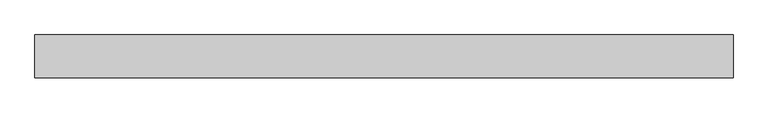
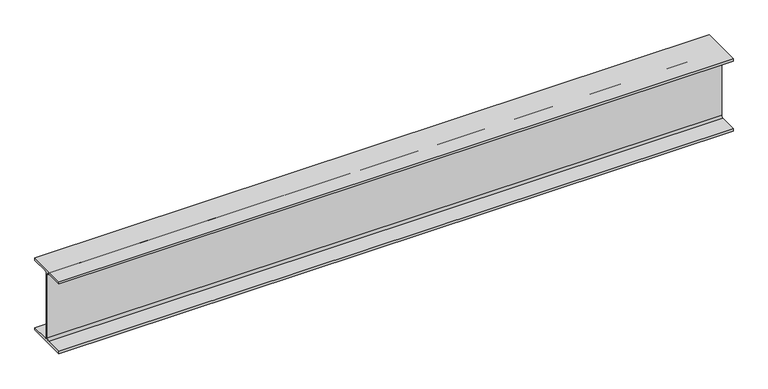
"""IFC4 building model written with IfcOpenShell, lengths in millimetres: beam geometry, Old_Steel Beam_H-KSD3502 : H_SB_ASB_H-250×125x6x9."""

import ifcopenshell
import ifcopenshell.guid

model = None  # the IFC model being written
_history = None  # IfcOwnerHistory: only IFC2X3 demands one
_inside = {}  # id of a spatial element -> (the spatial element, [elements in it])
_under = {}  # id of a project, library or spatial element -> (it, [spatial elements below it])
_declared = {}  # id of a project -> (the project, [libraries it declares])
_typed = {}  # id of a type object -> (the type object, [elements of that type])
_made_of = {}  # id of a material, layer set ... -> (it, [elements and type objects made of it])


def new_model(schema):
    """Start an empty IFC model of exactly this schema.

    Asked for "IFC4X3", IfcOpenShell would pick the latest addendum, in which some entities
    have other attributes; the version numbers below select the first issue.
    IFC2X3 requires an IfcOwnerHistory on every rooted entity: one is made here for all.
    """
    global model, _history
    if schema == "IFC4X3":
        model = ifcopenshell.file(schema_version=(4, 3, 0, 0))
    else:
        model = ifcopenshell.file(schema=schema)
    _inside.clear()
    _under.clear()
    _declared.clear()
    _typed.clear()
    _made_of.clear()
    _history = None
    if model.schema == "IFC2X3":
        org = make("IfcOrganization", Name="unknown")
        user = make(
            "IfcPersonAndOrganization",
            ThePerson=make("IfcPerson", FamilyName="unknown"),
            TheOrganization=org,
        )
        app = make(
            "IfcApplication",
            ApplicationDeveloper=org,
            Version="unknown",
            ApplicationFullName="unknown",
            ApplicationIdentifier="unknown",
        )
        _history = make(
            "IfcOwnerHistory",
            OwningUser=user,
            OwningApplication=app,
            ChangeAction="ADDED",
            CreationDate=0,
        )
    return model


def make(cls, **values):
    """One entity of the class cls with the attributes given. An attribute that is None is left unset."""
    return model.create_entity(
        cls, **{name: value for name, value in values.items() if value is not None}
    )


def rooted(cls, **values):
    """An entity with a GlobalId (a new one), such as an element, a storey or a relation."""
    return make(cls, GlobalId=ifcopenshell.guid.new(), OwnerHistory=_history, **values)


def si_unit(unit_type, name, prefix=None):
    """IfcSIUnit, for example si_unit("LENGTHUNIT", "METRE", prefix="MILLI")."""
    return make("IfcSIUnit", UnitType=unit_type, Prefix=prefix, Name=name)


def assignment(units):
    """IfcUnitAssignment: the units of a project."""
    return None if units is None else make("IfcUnitAssignment", Units=units)


def point(xyz):
    """IfcCartesianPoint."""
    return None if xyz is None else make("IfcCartesianPoint", Coordinates=xyz)


def direction(xyz):
    """IfcDirection."""
    return None if xyz is None else make("IfcDirection", DirectionRatios=xyz)


def frame(location, z_axis=None, x_axis=None):
    """IfcAxis2Placement3D, a coordinate frame: its origin and axes. An axis left out is left unset."""
    return make(
        "IfcAxis2Placement3D",
        Location=point(location),
        Axis=direction(z_axis),
        RefDirection=direction(x_axis),
    )


def frame_2d(location, x_axis=None):
    """IfcAxis2Placement2D, a coordinate frame in the plane: its origin and x axis."""
    return make(
        "IfcAxis2Placement2D", Location=point(location), RefDirection=direction(x_axis)
    )


def origin():
    """The frame at (0, 0, 0) with its axes left unset."""
    return frame((0.0, 0.0, 0.0))


def place(relative_to, where):
    """IfcLocalPlacement: puts the frame where relative to a parent placement (None: the world)."""
    return make(
        "IfcLocalPlacement", PlacementRelTo=relative_to, RelativePlacement=where
    )


def context(
    kind, dimensions, precision=None, world=None, true_north=None, identifier=None
):
    """IfcGeometricRepresentationContext, for example the 3D "Model" context."""
    return make(
        "IfcGeometricRepresentationContext",
        ContextIdentifier=identifier,
        ContextType=kind,
        CoordinateSpaceDimension=dimensions,
        Precision=precision,
        WorldCoordinateSystem=world,
        TrueNorth=true_north,
    )


def project(units=None, contexts=None):
    """IfcProject with its units and contexts."""
    return rooted(
        "IfcProject",
        Name="project",
        RepresentationContexts=contexts,
        UnitsInContext=assignment(units),
    )


def spatial(cls, under=None, at=None, **own):
    """A site, building, storey or space (cls), placed at a placement, below another one or the project."""
    s = rooted(cls, ObjectPlacement=at, **own)
    if under is not None:
        _under.setdefault(under.id(), (under, []))[1].append(s)
    return s


def polyline(points):
    """IfcPolyline through the points."""
    return make("IfcPolyline", Points=[point(p) for p in points])


def circle_curve(where, radius):
    """IfcCircle in the frame where."""
    return make("IfcCircle", Position=where, Radius=radius)


def trimmed(basis, trim1, trim2, sense, master):
    """IfcTrimmedCurve: the piece of a basis curve between two trims."""
    return make(
        "IfcTrimmedCurve",
        BasisCurve=basis,
        Trim1=trim1,
        Trim2=trim2,
        SenseAgreement=sense,
        MasterRepresentation=master,
    )


def segment(curve, same_sense, transition):
    """IfcCompositeCurveSegment."""
    return make(
        "IfcCompositeCurveSegment",
        Transition=transition,
        SameSense=same_sense,
        ParentCurve=curve,
    )


def composite_curve(segments, self_intersect=None):
    """IfcCompositeCurve: segments joined end to end."""
    return make("IfcCompositeCurve", Segments=segments, SelfIntersect=self_intersect)


def outline(outer, holes=None, kind="AREA"):
    """IfcArbitraryClosedProfileDef: a profile drawn as a closed curve; with holes, ...WithVoids."""
    if holes is None:
        return make("IfcArbitraryClosedProfileDef", ProfileType=kind, OuterCurve=outer)
    return make(
        "IfcArbitraryProfileDefWithVoids",
        ProfileType=kind,
        OuterCurve=outer,
        InnerCurves=holes,
    )


def extrude(swept, where, along, depth):
    """IfcExtrudedAreaSolid: the profile swept, set in the frame where, extruded along a direction by depth."""
    return make(
        "IfcExtrudedAreaSolid",
        SweptArea=swept,
        Position=where,
        ExtrudedDirection=direction(along),
        Depth=depth,
    )


def shape(context_of_items, identifier, shape_type, items):
    """IfcShapeRepresentation: the items that make up one representation, for example the "Body"."""
    return make(
        "IfcShapeRepresentation",
        ContextOfItems=context_of_items,
        RepresentationIdentifier=identifier,
        RepresentationType=shape_type,
        Items=items,
    )


def source(mapping_origin, context_of_items, identifier, shape_type, items):
    """IfcRepresentationMap: a shape defined once, which mapped items show again and again."""
    return make(
        "IfcRepresentationMap",
        MappingOrigin=mapping_origin,
        MappedRepresentation=shape(context_of_items, identifier, shape_type, items),
    )


def transform(
    local_origin,
    x_axis=None,
    y_axis=None,
    z_axis=None,
    scale=None,
    scale2=None,
    scale3=None,
    uniform=True,
):
    """IfcCartesianTransformationOperator3D, or its non-uniform kind. x_axis, y_axis, z_axis: its Axis1, 2, 3."""
    if uniform:
        return make(
            "IfcCartesianTransformationOperator3D",
            Axis1=direction(x_axis),
            Axis2=direction(y_axis),
            LocalOrigin=point(local_origin),
            Scale=scale,
            Axis3=direction(z_axis),
        )
    return make(
        "IfcCartesianTransformationOperator3DnonUniform",
        Axis1=direction(x_axis),
        Axis2=direction(y_axis),
        LocalOrigin=point(local_origin),
        Scale=scale,
        Axis3=direction(z_axis),
        Scale2=scale2,
        Scale3=scale3,
    )


def mapped(mapping_source, mapping_target):
    """IfcMappedItem: shows the shape of a source again, moved by a transform."""
    return make(
        "IfcMappedItem", MappingSource=mapping_source, MappingTarget=mapping_target
    )


def made_of(thing, what):
    """Note that an element or type object is made of a material, layer set ...; save() writes the relation."""
    if what is not None:
        _made_of.setdefault(what.id(), (what, []))[1].append(thing)
    return thing


def element(
    cls,
    number,
    at=None,
    inside=None,
    cuts=None,
    type_object=None,
    material=None,
    context=None,
    identifier="Body",
    shape_type=None,
    held_by="IfcProductDefinitionShape",
    body=None,
    shapes=None,
    **own,
):
    """One element of the class cls, such as IfcWall. Its Tag is "e" and its number.

    at: its placement. inside: the storey or other place that contains it. cuts: it is an
    opening in that element (IfcRelVoidsElement). A single representation is given by context,
    identifier, shape_type and body (its items); several are given by shapes. held_by: the class
    of the entity that holds the representations. save() writes the other relations.
    """
    e = rooted(cls, Tag="e%d" % number, ObjectPlacement=at, **own)
    if body is not None:
        shapes = [shape(context, identifier, shape_type, body)]
    if shapes is not None:
        e.Representation = make(held_by, Representations=shapes)
    if inside is not None:
        _inside.setdefault(inside.id(), (inside, []))[1].append(e)
    if cuts is not None:
        rooted(
            "IfcRelVoidsElement", RelatingBuildingElement=cuts, RelatedOpeningElement=e
        )
    if type_object is not None:
        _typed.setdefault(type_object.id(), (type_object, []))[1].append(e)
    return made_of(e, material)


def aggregate(whole, parts):
    """IfcRelAggregates: a whole, such as a stair, and the parts it consists of."""
    return rooted("IfcRelAggregates", RelatingObject=whole, RelatedObjects=parts)


def save(model, path):
    """Write the relations noted so far, then the file.

    IfcRelAggregates (storeys below a building ...), IfcRelContainedInSpatialStructure (elements
    in a storey), IfcRelDefinesByType, IfcRelAssociatesMaterial and IfcRelDeclares: one each for
    every whole, place, type object, material and project.
    """
    for whole, parts in _under.values():
        aggregate(whole, parts)
    for where, things in _inside.values():
        rooted(
            "IfcRelContainedInSpatialStructure",
            RelatedElements=things,
            RelatingStructure=where,
        )
    for kind, things in _typed.values():
        rooted("IfcRelDefinesByType", RelatedObjects=things, RelatingType=kind)
    for what, things in _made_of.values():
        rooted("IfcRelAssociatesMaterial", RelatedObjects=things, RelatingMaterial=what)
    for by, libraries in _declared.values():
        rooted("IfcRelDeclares", RelatingContext=by, RelatedDefinitions=libraries)
    model.write(path)


def beam_119fac50(model_context):
    return source(origin(), model_context, "Body", "SweptSolid", [
        extrude(outline(composite_curve([segment(polyline([(82.5, -141.5), (82.5, -151.7), (-82.5, -151.7), (-82.5, -141.5), (-11.9, -141.5)]), True, "CONTINUOUS"), segment(trimmed(circle_curve(frame_2d((-11.9, -132.6)), 8.9), [point((-11.9, -141.5))], [point((-3.0, -132.6))], True, "CARTESIAN"), True, "CONTINUOUS"), segment(polyline([(-3.0, -132.6), (-3.0, 132.6)]), True, "CONTINUOUS"), segment(trimmed(circle_curve(frame_2d((-11.9, 132.6)), 8.9), [point((-3.0, 132.6))], [point((-11.9, 141.5))], True, "CARTESIAN"), True, "CONTINUOUS"), segment(polyline([(-11.9, 141.5), (-82.5, 141.5), (-82.5, 151.7), (82.5, 151.7), (82.5, 141.5), (11.9, 141.5)]), True, "CONTINUOUS"), segment(trimmed(circle_curve(frame_2d((11.9, 132.6)), 8.9), [point((11.9, 141.5))], [point((3.0, 132.6))], True, "CARTESIAN"), True, "CONTINUOUS"), segment(polyline([(3.0, 132.6), (3.0, -132.6)]), True, "CONTINUOUS"), segment(trimmed(circle_curve(frame_2d((11.9, -132.6)), 8.9), [point((3.0, -132.6))], [point((11.9, -141.5))], True, "CARTESIAN"), True, "CONTINUOUS"), segment(polyline([(11.9, -141.5), (82.5, -141.5)]), True, "CONTINUOUS")], self_intersect=False)), frame((-1404.8000503, 0.0, 0.0), z_axis=(1.0, 0.0, 0.0), x_axis=(0.0, 1.0, 0.0)), (0.0, 0.0, 1.0), 2674.6999215),
    ])


if __name__ == "__main__":
    model = new_model("IFC4")
    model_context = context("Model", 3, world=origin())
    ifc_project = project(units=[si_unit("LENGTHUNIT", "METRE", prefix="MILLI")], contexts=[model_context])
    site = spatial("IfcSite", under=ifc_project)
    building = spatial("IfcBuilding", under=site)
    placement = place(None, origin())
    beam_shape = beam_119fac50(model_context)
    element("IfcBeam", 1, ObjectType="Old_Steel Beam_H-KSD3502 : H_SB_ASB_H-250×125x6x9", at=placement, inside=building, context=model_context, shape_type="MappedRepresentation", body=[
        mapped(beam_shape, transform((0.0, 0.0, 0.0), x_axis=(1.0, 0.0, 0.0), y_axis=(0.0, 1.0, 0.0), z_axis=(0.0, 0.0, 1.0))),
    ])
    save(model, "model.ifc")

# Revit data of these elements
# Type "Old_Steel Beam_H-KSD3502 : H_SB_ASB_H-250×125x6x9"
#   Width = 12.5 cm
#   Web Thickness = 0.6 cm
#   Web Fillet = 1.2 cm
#   Warping Constant = 42539.8 cm⁶
#   Torsional Moment of Inertia = 7.8102 cm⁴
#   Torsional Modulus = 1.0 cm³
#   Section Area = 37.66 cm²
#   Plastic Modulus weak axis = 73.1 cm³
#   Plastic Modulus strong axis = 366.0 cm³
#   Perimeter = 0.97 m²/m
#   Nominal Weight = 29.60 kgf/m
#   Moment of Inertia weak axis = 294.00 cm⁴
#   Moment of Inertia strong axis = 4050.00 cm⁴
#   Height = 25.0 cm
#   Flange Thickness = 0.9 cm
#   Elastic Modulus weak axis = 47.0 cm³
#   Elastic Modulus strong axis = 324.0 cm³
#   Centroid Vertical = 12.5 cm
#   Centroid Horizontal = 6.25 cm
#   Length [instance default] = 1.5240 m
#   Structural Material [instance default] = Steel, 45-345
#   Assembly Code = ""
# Element 1 (IfcBeam, "Old_Steel Beam_H-KSD3502 : H_SB_ASB_H-250×125x6x9")
#   Structural Material = none
# Materials
#   "Steel, 45-345": class "Metal", colour RGB 189 187 185, transparency 0, Description = "Steel 345 MPa", Cost = 0
